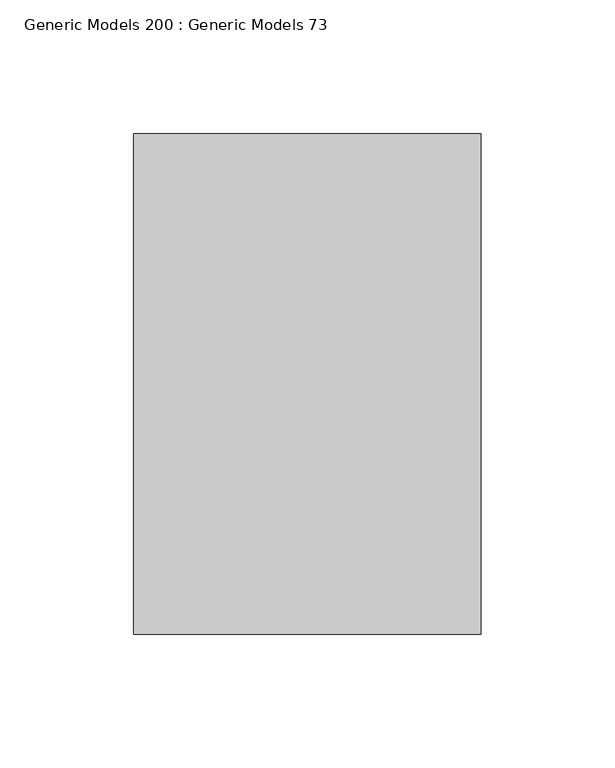
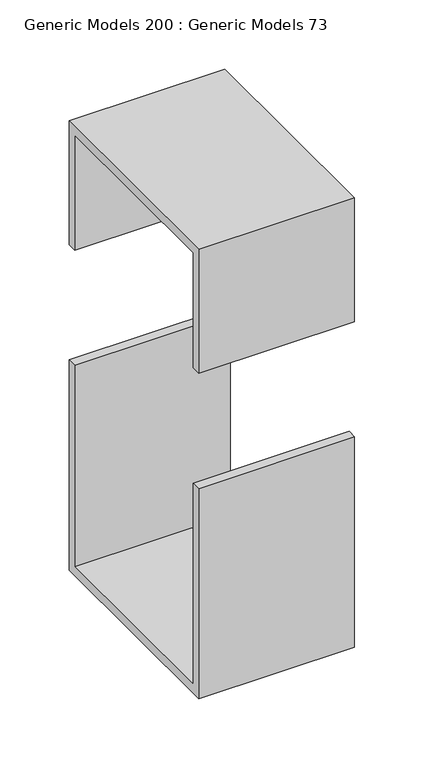
"""IFC4 building model written with IfcOpenShell, lengths in millimetres: proxy geometry, Generic Models 200 : Generic Models 73."""

from ifc_helpers import new_model, si_unit, frame, origin, place, context, project, spatial, polyline, outline, extrude, source, transform, mapped, element, save


def generic_models_200_generic_models_73_f198fd3d(model_context):
    return source(origin(), model_context, "Body", "SweptSolid", [
        extrude(outline(polyline([(36493.1457942, 268757.4), (36493.1457942, 268935.2), (36501.0832942, 268935.2), (36501.0832942, 268749.4625), (36313.7582942, 268749.4625), (36313.7582942, 268935.2), (36321.6957942, 268935.2), (36321.6957942, 268757.4), (36493.1457942, 268757.4)])), frame((31910.3221032, 0.0, 0.0), z_axis=(1.0, 0.0, 0.0), x_axis=(0.0, 1.0, 0.0)), (0.0, 0.0, 1.0), 130.175),
        extrude(outline(polyline([(36493.1457942, 269138.4), (36321.6957942, 269138.4), (36321.6957942, 269036.8), (36313.7582942, 269036.8), (36313.7582942, 269146.3375), (36501.0832942, 269146.3375), (36501.0832942, 269036.8), (36493.1457942, 269036.8), (36493.1457942, 269138.4)])), frame((31910.3221032, 0.0, 0.0), z_axis=(1.0, 0.0, 0.0), x_axis=(0.0, 1.0, 0.0)), (0.0, 0.0, 1.0), 130.175),
    ])


if __name__ == "__main__":
    model = new_model("IFC4")
    model_context = context("Model", 3, world=origin())
    ifc_project = project(units=[si_unit("LENGTHUNIT", "METRE", prefix="MILLI")], contexts=[model_context])
    site = spatial("IfcSite", under=ifc_project)
    building = spatial("IfcBuilding", under=site)
    placement = place(None, origin())
    generic_models_200_generic_models_73_shape = generic_models_200_generic_models_73_f198fd3d(model_context)
    element("IfcBuildingElementProxy", 1, Name="Generic Models 200 : Generic Models 73", ObjectType="Generic Models 200 : Generic Models 73", at=placement, inside=building, context=model_context, shape_type="MappedRepresentation", body=[
        mapped(generic_models_200_generic_models_73_shape, transform((0.0, 0.0, 0.0), x_axis=(1.0, 0.0, 0.0), y_axis=(0.0, 1.0, 0.0), z_axis=(0.0, 0.0, 1.0))),
    ])
    save(model, "model.ifc")

# Revit data of these elements
# Element 1 (IfcBuildingElementProxy, "Generic Models 200 : Generic Models 73")
#   Materials on its faces: "5/16 BENT PLATE SADDLE \nW/ 2 1\"DIA. THRU BOLTS"
# Materials
#   "5/16 BENT PLATE SADDLE \nW/ 2 1\"DIA. THRU BOLTS": class "Metal", colour RGB 199 199 199, transparency 0, Description = "Carbon steel", Cost = 0
